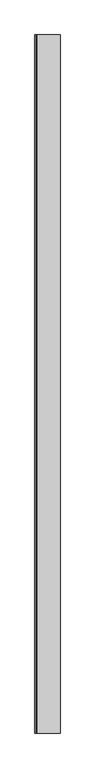
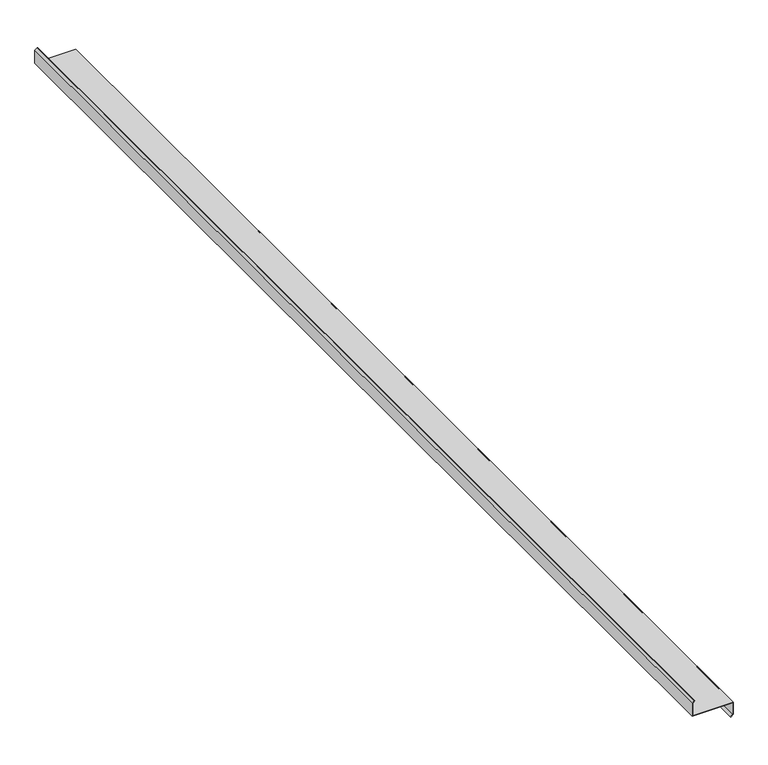
"""IFC4 building model written with IfcOpenShell, lengths in millimetres: proxy geometry, Generic Models 7:Generic Models 1:1:Generic Models 1:1 : Generic Models 7:Generic Models 1:337419:35 : Generic Models 7:Generic Models 1:1:Generic Models 1:1 : Generic Models 7:Generic Models 1:337419:306201."""

from ifc_helpers import new_model, si_unit, frame, origin, place, context, project, spatial, polyline, outline, extrude, source, transform, mapped, element, save


def generic_models_7138f307(model_context):
    return source(origin(), model_context, "Body", "SweptSolid", [
        extrude(outline(polyline([(3588.1924559, 667530.7466425), (3586.2205211, 667532.7185773), (3598.465625, 667547.3117239), (3677.8406249, 667547.3117239), (3677.8406249, 667296.0898489), (3759.492039, 667296.0898489), (3770.9044367, 667309.6906149), (3773.0326039, 667307.9048706), (3760.7874999, 667293.3117239), (3675.0624999, 667293.3117239), (3675.0624999, 667544.533599), (3599.761086, 667544.533599), (3588.1924559, 667530.7466425)])), frame((0.0, -571669.6163841, 0.0), z_axis=(0.0, 1.0, 0.0), x_axis=(0.0, 0.0, 1.0)), (0.0, 0.0, 1.0), 7061.2),
    ])


if __name__ == "__main__":
    model = new_model("IFC4")
    model_context = context("Model", 3, world=origin())
    ifc_project = project(units=[si_unit("LENGTHUNIT", "METRE", prefix="MILLI")], contexts=[model_context])
    site = spatial("IfcSite", under=ifc_project)
    building = spatial("IfcBuilding", under=site)
    placement = place(None, origin())
    generic_models_shape = generic_models_7138f307(model_context)
    element("IfcBuildingElementProxy", 1, Name="Generic Models 7:Generic Models 1:1:Generic Models 1:1 : Generic Models 7:Generic Models 1:337419:35 : Generic Models 7:Generic Models 1:1:Generic Models 1:1 : Generic Models 7:Generic Models 1:337419:306201", ObjectType="Generic Models 7:Generic Models 1:1:Generic Models 1:1 : Generic Models 7:Generic Models 1:337419:35 : Generic Models 7:Generic Models 1:1:Generic Models 1:1 : Generic Models 7:Generic Models 1:337419:306201", at=placement, inside=building, context=model_context, shape_type="MappedRepresentation", body=[
        mapped(generic_models_shape, transform((0.0, 0.0, 0.0), x_axis=(1.0, 0.0, 0.0), y_axis=(0.0, 1.0, 0.0), z_axis=(0.0, 0.0, 1.0))),
    ])
    save(model, "model.ifc")

# Revit data of these elements
# Type "Generic Models 7:Generic Models 1:1:Generic Models 1:1 : Generic Models 7:Generic Models 1:337419:35 : Generic Models 7:Generic Models 1:1:Generic Models 1:1 : Generic Models 7:Generic Models 1:337419:306201"
#   NameOverride = "Generic Models 7:Generic Models 1:1:Generic Models 1:1 : Generic Models 7:Generic Models 1:337419:306201"
#   ObjectTypeOverride = "Generic Models 1:1 : Generic Models 7:Generic Models 1:337419"
#   Reference = "Generic Models 1"
#   Tag = "306201"
# Element 1 (IfcBuildingElementProxy, "Generic Models 7:Generic Models 1:1:Generic Models 1:1 : Generic Models 7:Generic Models 1:337419:35 : Generic Models 7:Generic Models 1:1:Generic Models 1:1 : Generic Models 7:Generic Models 1:337419:306201")
#   Materials on its faces: "CEE' SECTION (8.0x3.5C - SEE STRUCT. DWGS)"
# Materials
#   "CEE' SECTION (8.0x3.5C - SEE STRUCT. DWGS)": class "Unassigned", colour RGB 210 209 208, transparency 0, Keynote = "M05121300.02", Cost = 0
